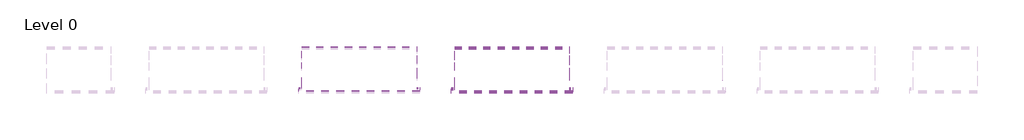
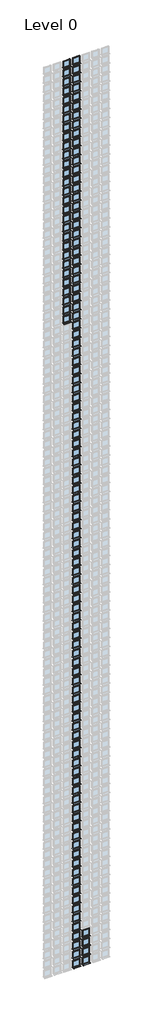
# One storey, part 12 of 75: 133 windows.
# Revit data of these elements (continued)
# Project information
#   Project Issue Date = "Issue Date"
#   Project Status = "Project Status"
#   Client Name = "Owner"
#   Project Address = "Enter address here"
#   Project Name = "Project Name"
#   Project Number = "Project Number"
# Type "Windows_Sgl_Plain : Square Green"
#   Type Mark = "51"
#   Operation = "SinglePanel"
#   Construction Type Id = "SGL"
#   Manufacturer = "Revit"
#   Keynote = "L10"
#   Analytic Construction = "Large single-glazed windows"
#   Wrap Layers (Ext) from Ext = 102.5 mm
#   Wrap Layers (Int) from Ext = 177.5 mm
#   Window Board Projection = 25 mm
#   Window Board Extension = 25 mm
#   Visual Light Transmittance = 0.9
#   Solar Heat Gain Coefficient = 0.86
#   Rough Width = 910 mm
#   Rough Height = 910 mm
#   Height = 910 mm
#   Width = 910 mm
#   Heat Transfer Coefficient (U) = 5.5617 W/(m²·K)
#   Glazing Thickness = 24 mm
#   FrameOffset - External = 50 mm
#   Frame Depth = 65 mm
#   Default Head Height = 2110 mm
#   Cill Depth = 87.5 mm
#   Cavity Closer Width = 50 mm
#   Cavity Closer Offset from Ext = 102.5 mm
#   Cavity Closer Depth = 85 mm
#   Vis - Cavity Closers = yes
#   Material Trim = Window Frame
#   Material Glass = Green Glass
#   Material Frame = Window Frame
#   Wall Closure = (empty or 0)
# Type "Windows_Sgl_Plain : Square Normal"
#   Type Mark = "44"
#   Operation = "SinglePanel"
#   Construction Type Id = "SGL"
#   Manufacturer = "Revit"
#   Keynote = "L10"
#   Analytic Construction = "Large single-glazed windows"
#   Wrap Layers (Ext) from Ext = 102.5 mm
#   Wrap Layers (Int) from Ext = 177.5 mm
#   Window Board Projection = 25 mm
#   Window Board Extension = 25 mm
#   Visual Light Transmittance = 0.9
#   Solar Heat Gain Coefficient = 0.86
#   Rough Width = 910 mm
#   Rough Height = 910 mm
#   Height = 910 mm
#   Width = 910 mm
#   Heat Transfer Coefficient (U) = 5.5617 W/(m²·K)
#   Glazing Thickness = 24 mm
#   FrameOffset - External = 50 mm
#   Frame Depth = 65 mm
#   Default Head Height = 2110 mm
#   Cill Depth = 87.5 mm
#   Cavity Closer Width = 50 mm
#   Cavity Closer Offset from Ext = 102.5 mm
#   Cavity Closer Depth = 85 mm
#   Vis - Cavity Closers = yes
#   Material Trim = Window Frame
#   Material Glass = Glass
#   Material Frame = Window Frame
#   Wall Closure = (empty or 0)
# Type "Windows_Sgl_Plain : Square Red"
#   Type Mark = "50"
#   Operation = "SinglePanel"
#   Construction Type Id = "SGL"
#   Manufacturer = "Revit"
#   Keynote = "L10"
#   Analytic Construction = "Large single-glazed windows"
#   Wrap Layers (Ext) from Ext = 102.5 mm
#   Wrap Layers (Int) from Ext = 177.5 mm
#   Window Board Projection = 25 mm
#   Window Board Extension = 25 mm
#   Visual Light Transmittance = 0.9
#   Solar Heat Gain Coefficient = 0.86
#   Rough Width = 910 mm
#   Rough Height = 910 mm
#   Height = 910 mm
#   Width = 910 mm
#   Heat Transfer Coefficient (U) = 5.5617 W/(m²·K)
#   Glazing Thickness = 24 mm
#   FrameOffset - External = 50 mm
#   Frame Depth = 65 mm
#   Default Head Height = 2110 mm
#   Cill Depth = 87.5 mm
#   Cavity Closer Width = 50 mm
#   Cavity Closer Offset from Ext = 102.5 mm
#   Cavity Closer Depth = 85 mm
#   Vis - Cavity Closers = yes
#   Material Trim = Window Frame
#   Material Glass = Red Glass
#   Material Frame = Window Frame
#   Wall Closure = (empty or 0)
# Element 1 (IfcWindow, "Windows_Sgl_Plain : Square Green")
#   Mark = "6458"
#   Phase Created = New Construction
#   Materials on its faces: "Window Frame", "Green Glass"
# Element 2 (IfcWindow, "Windows_Sgl_Plain : Square Green")
#   Mark = "12457"
#   Phase Created = New Construction
#   Materials on its faces: "Window Frame", "Green Glass"
# Element 3 (IfcWindow, "Windows_Sgl_Plain : Square Green")
#   Mark = "12557"
#   Phase Created = New Construction
#   Materials on its faces: "Window Frame", "Green Glass"
# Element 4 (IfcWindow, "Windows_Sgl_Plain : Square Normal")
#   Mark = "6457"
#   Phase Created = New Construction
#   Materials on its faces: "Window Frame", "Glass"
# Element 5 (IfcWindow, "Windows_Sgl_Plain : Square Normal")
#   Mark = "6557"
#   Phase Created = New Construction
#   Materials on its faces: "Window Frame", "Glass"
# Element 6 (IfcWindow, "Windows_Sgl_Plain : Square Normal")
#   Mark = "6558"
#   Phase Created = New Construction
#   Materials on its faces: "Window Frame", "Glass"
# Element 7 (IfcWindow, "Windows_Sgl_Plain : Square Normal")
#   Mark = "6657"
#   Phase Created = New Construction
#   Materials on its faces: "Window Frame", "Glass"
# Element 8 (IfcWindow, "Windows_Sgl_Plain : Square Normal")
#   Mark = "6757"
#   Phase Created = New Construction
#   Materials on its faces: "Window Frame", "Glass"
# Element 9 (IfcWindow, "Windows_Sgl_Plain : Square Normal")
#   Mark = "6857"
#   Phase Created = New Construction
#   Materials on its faces: "Window Frame", "Glass"
# Element 10 (IfcWindow, "Windows_Sgl_Plain : Square Normal")
#   Mark = "6957"
#   Phase Created = New Construction
#   Materials on its faces: "Window Frame", "Glass"
# Element 11 (IfcWindow, "Windows_Sgl_Plain : Square Normal")
#   Mark = "7057"
#   Phase Created = New Construction
#   Materials on its faces: "Window Frame", "Glass"
# Element 12 (IfcWindow, "Windows_Sgl_Plain : Square Normal")
#   Mark = "7157"
#   Phase Created = New Construction
#   Materials on its faces: "Window Frame", "Glass"
# Element 13 (IfcWindow, "Windows_Sgl_Plain : Square Normal")
#   Mark = "7257"
#   Phase Created = New Construction
#   Materials on its faces: "Window Frame", "Glass"
# Element 14 (IfcWindow, "Windows_Sgl_Plain : Square Normal")
#   Mark = "7357"
#   Phase Created = New Construction
#   Materials on its faces: "Window Frame", "Glass"
# Element 15 (IfcWindow, "Windows_Sgl_Plain : Square Normal")
#   Mark = "7457"
#   Phase Created = New Construction
#   Materials on its faces: "Window Frame", "Glass"
# Element 16 (IfcWindow, "Windows_Sgl_Plain : Square Normal")
#   Mark = "7557"
#   Phase Created = New Construction
#   Materials on its faces: "Window Frame", "Glass"
# Element 17 (IfcWindow, "Windows_Sgl_Plain : Square Normal")
#   Mark = "7657"
#   Phase Created = New Construction
#   Materials on its faces: "Window Frame", "Glass"
# Element 18 (IfcWindow, "Windows_Sgl_Plain : Square Normal")
#   Mark = "7757"
#   Phase Created = New Construction
#   Materials on its faces: "Window Frame", "Glass"
# Element 19 (IfcWindow, "Windows_Sgl_Plain : Square Normal")
#   Mark = "7857"
#   Phase Created = New Construction
#   Materials on its faces: "Window Frame", "Glass"
# Element 20 (IfcWindow, "Windows_Sgl_Plain : Square Normal")
#   Mark = "7957"
#   Phase Created = New Construction
#   Materials on its faces: "Window Frame", "Glass"
# Element 21 (IfcWindow, "Windows_Sgl_Plain : Square Normal")
#   Mark = "8057"
#   Phase Created = New Construction
#   Materials on its faces: "Window Frame", "Glass"
# Element 22 (IfcWindow, "Windows_Sgl_Plain : Square Normal")
#   Mark = "8157"
#   Phase Created = New Construction
#   Materials on its faces: "Window Frame", "Glass"
# Element 23 (IfcWindow, "Windows_Sgl_Plain : Square Normal")
#   Mark = "8257"
#   Phase Created = New Construction
#   Materials on its faces: "Window Frame", "Glass"
# Element 24 (IfcWindow, "Windows_Sgl_Plain : Square Normal")
#   Mark = "8357"
#   Phase Created = New Construction
#   Materials on its faces: "Window Frame", "Glass"
# Element 25 (IfcWindow, "Windows_Sgl_Plain : Square Normal")
#   Mark = "8457"
#   Phase Created = New Construction
#   Materials on its faces: "Window Frame", "Glass"
# Element 26 (IfcWindow, "Windows_Sgl_Plain : Square Normal")
#   Mark = "8557"
#   Phase Created = New Construction
#   Materials on its faces: "Window Frame", "Glass"
# Element 27 (IfcWindow, "Windows_Sgl_Plain : Square Normal")
#   Mark = "8657"
#   Phase Created = New Construction
#   Materials on its faces: "Window Frame", "Glass"
# Element 28 (IfcWindow, "Windows_Sgl_Plain : Square Normal")
#   Mark = "8757"
#   Phase Created = New Construction
#   Materials on its faces: "Window Frame", "Glass"
# Element 29 (IfcWindow, "Windows_Sgl_Plain : Square Normal")
#   Mark = "8857"
#   Phase Created = New Construction
#   Materials on its faces: "Window Frame", "Glass"
# Element 30 (IfcWindow, "Windows_Sgl_Plain : Square Normal")
#   Mark = "8957"
#   Phase Created = New Construction
#   Materials on its faces: "Window Frame", "Glass"
# Element 31 (IfcWindow, "Windows_Sgl_Plain : Square Normal")
#   Mark = "9057"
#   Phase Created = New Construction
#   Materials on its faces: "Window Frame", "Glass"
# Element 32 (IfcWindow, "Windows_Sgl_Plain : Square Normal")
#   Mark = "9157"
#   Phase Created = New Construction
#   Materials on its faces: "Window Frame", "Glass"
# Element 33 (IfcWindow, "Windows_Sgl_Plain : Square Normal")
#   Mark = "9257"
#   Phase Created = New Construction
#   Materials on its faces: "Window Frame", "Glass"
# Element 34 (IfcWindow, "Windows_Sgl_Plain : Square Normal")
#   Mark = "9357"
#   Phase Created = New Construction
#   Materials on its faces: "Window Frame", "Glass"
# Element 35 (IfcWindow, "Windows_Sgl_Plain : Square Normal")
#   Mark = "9457"
#   Phase Created = New Construction
#   Materials on its faces: "Window Frame", "Glass"
# Element 36 (IfcWindow, "Windows_Sgl_Plain : Square Normal")
#   Mark = "9557"
#   Phase Created = New Construction
#   Materials on its faces: "Window Frame", "Glass"
# Element 37 (IfcWindow, "Windows_Sgl_Plain : Square Normal")
#   Mark = "9657"
#   Phase Created = New Construction
#   Materials on its faces: "Window Frame", "Glass"
# Element 38 (IfcWindow, "Windows_Sgl_Plain : Square Normal")
#   Mark = "9757"
#   Phase Created = New Construction
#   Materials on its faces: "Window Frame", "Glass"
# Element 39 (IfcWindow, "Windows_Sgl_Plain : Square Normal")
#   Mark = "9857"
#   Phase Created = New Construction
#   Materials on its faces: "Window Frame", "Glass"
# Element 40 (IfcWindow, "Windows_Sgl_Plain : Square Normal")
#   Mark = "9957"
#   Phase Created = New Construction
#   Materials on its faces: "Window Frame", "Glass"
# Element 41 (IfcWindow, "Windows_Sgl_Plain : Square Normal")
#   Mark = "10057"
#   Phase Created = New Construction
#   Materials on its faces: "Window Frame", "Glass"
# Element 42 (IfcWindow, "Windows_Sgl_Plain : Square Normal")
#   Mark = "10157"
#   Phase Created = New Construction
#   Materials on its faces: "Window Frame", "Glass"
# Element 43 (IfcWindow, "Windows_Sgl_Plain : Square Normal")
#   Mark = "10257"
#   Phase Created = New Construction
#   Materials on its faces: "Window Frame", "Glass"
# Element 44 (IfcWindow, "Windows_Sgl_Plain : Square Normal")
#   Mark = "10357"
#   Phase Created = New Construction
#   Materials on its faces: "Window Frame", "Glass"
# Element 45 (IfcWindow, "Windows_Sgl_Plain : Square Normal")
#   Mark = "10457"
#   Phase Created = New Construction
#   Materials on its faces: "Window Frame", "Glass"
# Element 46 (IfcWindow, "Windows_Sgl_Plain : Square Normal")
#   Mark = "10557"
#   Phase Created = New Construction
#   Materials on its faces: "Window Frame", "Glass"
# Element 47 (IfcWindow, "Windows_Sgl_Plain : Square Normal")
#   Mark = "11057"
#   Phase Created = New Construction
#   Materials on its faces: "Window Frame", "Glass"
# Element 48 (IfcWindow, "Windows_Sgl_Plain : Square Normal")
#   Mark = "11157"
#   Phase Created = New Construction
#   Materials on its faces: "Window Frame", "Glass"
# Element 49 (IfcWindow, "Windows_Sgl_Plain : Square Normal")
#   Mark = "11257"
#   Phase Created = New Construction
#   Materials on its faces: "Window Frame", "Glass"
# Element 50 (IfcWindow, "Windows_Sgl_Plain : Square Normal")
#   Mark = "11357"
#   Phase Created = New Construction
#   Materials on its faces: "Window Frame", "Glass"
# Element 51 (IfcWindow, "Windows_Sgl_Plain : Square Normal")
#   Mark = "11457"
#   Phase Created = New Construction
#   Materials on its faces: "Window Frame", "Glass"
# Element 52 (IfcWindow, "Windows_Sgl_Plain : Square Normal")
#   Mark = "11557"
#   Phase Created = New Construction
#   Materials on its faces: "Window Frame", "Glass"
# Element 53 (IfcWindow, "Windows_Sgl_Plain : Square Normal")
#   Mark = "11657"
#   Phase Created = New Construction
#   Materials on its faces: "Window Frame", "Glass"
# Element 54 (IfcWindow, "Windows_Sgl_Plain : Square Normal")
#   Mark = "11757"
#   Phase Created = New Construction
#   Materials on its faces: "Window Frame", "Glass"
# Element 55 (IfcWindow, "Windows_Sgl_Plain : Square Normal")
#   Mark = "11857"
#   Phase Created = New Construction
#   Materials on its faces: "Window Frame", "Glass"
# Element 56 (IfcWindow, "Windows_Sgl_Plain : Square Normal")
#   Mark = "11957"
#   Phase Created = New Construction
#   Materials on its faces: "Window Frame", "Glass"
# Element 57 (IfcWindow, "Windows_Sgl_Plain : Square Normal")
#   Mark = "12057"
#   Phase Created = New Construction
#   Materials on its faces: "Window Frame", "Glass"
# Element 58 (IfcWindow, "Windows_Sgl_Plain : Square Normal")
#   Mark = "12157"
#   Phase Created = New Construction
#   Materials on its faces: "Window Frame", "Glass"
# Element 59 (IfcWindow, "Windows_Sgl_Plain : Square Normal")
#   Mark = "12257"
#   Phase Created = New Construction
#   Materials on its faces: "Window Frame", "Glass"
# Element 60 (IfcWindow, "Windows_Sgl_Plain : Square Normal")
#   Mark = "12357"
#   Phase Created = New Construction
#   Materials on its faces: "Window Frame", "Glass"
# Element 61 (IfcWindow, "Windows_Sgl_Plain : Square Normal")
#   Mark = "12657"
#   Phase Created = New Construction
#   Materials on its faces: "Window Frame", "Glass"
# Element 62 (IfcWindow, "Windows_Sgl_Plain : Square Normal")
#   Mark = "12757"
#   Phase Created = New Construction
#   Materials on its faces: "Window Frame", "Glass"
# Element 63 (IfcWindow, "Windows_Sgl_Plain : Square Normal")
#   Mark = "12857"
#   Phase Created = New Construction
#   Materials on its faces: "Window Frame", "Glass"
# Element 64 (IfcWindow, "Windows_Sgl_Plain : Square Normal")
#   Mark = "12957"
#   Phase Created = New Construction
#   Materials on its faces: "Window Frame", "Glass"
# Element 65 (IfcWindow, "Windows_Sgl_Plain : Square Normal")
#   Mark = "13057"
#   Phase Created = New Construction
#   Materials on its faces: "Window Frame", "Glass"
# Element 66 (IfcWindow, "Windows_Sgl_Plain : Square Normal")
#   Mark = "13157"
#   Phase Created = New Construction
#   Materials on its faces: "Window Frame", "Glass"
# Element 67 (IfcWindow, "Windows_Sgl_Plain : Square Normal")
#   Mark = "13257"
#   Phase Created = New Construction
#   Materials on its faces: "Window Frame", "Glass"
# Element 68 (IfcWindow, "Windows_Sgl_Plain : Square Normal")
#   Mark = "13356"
#   Phase Created = New Construction
#   Materials on its faces: "Window Frame", "Glass"
# Element 69 (IfcWindow, "Windows_Sgl_Plain : Square Normal")
#   Mark = "13357"
#   Phase Created = New Construction
#   Materials on its faces: "Window Frame", "Glass"
# Element 70 (IfcWindow, "Windows_Sgl_Plain : Square Normal")
#   Mark = "13456"
#   Phase Created = New Construction
#   Materials on its faces: "Window Frame", "Glass"
# Element 71 (IfcWindow, "Windows_Sgl_Plain : Square Normal")
#   Mark = "13457"
#   Phase Created = New Construction
#   Materials on its faces: "Window Frame", "Glass"
# Element 72 (IfcWindow, "Windows_Sgl_Plain : Square Normal")
#   Mark = "13556"
#   Phase Created = New Construction
#   Materials on its faces: "Window Frame", "Glass"
# Element 73 (IfcWindow, "Windows_Sgl_Plain : Square Normal")
#   Mark = "13557"
#   Phase Created = New Construction
#   Materials on its faces: "Window Frame", "Glass"
# Element 74 (IfcWindow, "Windows_Sgl_Plain : Square Normal")
#   Mark = "13656"
#   Phase Created = New Construction
#   Materials on its faces: "Window Frame", "Glass"
# Element 75 (IfcWindow, "Windows_Sgl_Plain : Square Normal")
#   Mark = "13657"
#   Phase Created = New Construction
#   Materials on its faces: "Window Frame", "Glass"
# Element 76 (IfcWindow, "Windows_Sgl_Plain : Square Normal")
#   Mark = "13756"
#   Phase Created = New Construction
#   Materials on its faces: "Window Frame", "Glass"
# Element 77 (IfcWindow, "Windows_Sgl_Plain : Square Normal")
#   Mark = "13757"
#   Phase Created = New Construction
#   Materials on its faces: "Window Frame", "Glass"
# Element 78 (IfcWindow, "Windows_Sgl_Plain : Square Normal")
#   Mark = "13856"
#   Phase Created = New Construction
#   Materials on its faces: "Window Frame", "Glass"
# Element 79 (IfcWindow, "Windows_Sgl_Plain : Square Normal")
#   Mark = "13857"
#   Phase Created = New Construction
#   Materials on its faces: "Window Frame", "Glass"
# Element 80 (IfcWindow, "Windows_Sgl_Plain : Square Normal")
#   Mark = "13956"
#   Phase Created = New Construction
#   Materials on its faces: "Window Frame", "Glass"
# Element 81 (IfcWindow, "Windows_Sgl_Plain : Square Normal")
#   Mark = "13957"
#   Phase Created = New Construction
#   Materials on its faces: "Window Frame", "Glass"
# Element 82 (IfcWindow, "Windows_Sgl_Plain : Square Normal")
#   Mark = "14056"
#   Phase Created = New Construction
#   Materials on its faces: "Window Frame", "Glass"
# Element 83 (IfcWindow, "Windows_Sgl_Plain : Square Normal")
#   Mark = "14057"
#   Phase Created = New Construction
#   Materials on its faces: "Window Frame", "Glass"
# Element 84 (IfcWindow, "Windows_Sgl_Plain : Square Normal")
#   Mark = "14156"
#   Phase Created = New Construction
#   Materials on its faces: "Window Frame", "Glass"
# Element 85 (IfcWindow, "Windows_Sgl_Plain : Square Normal")
#   Mark = "14157"
#   Phase Created = New Construction
#   Materials on its faces: "Window Frame", "Glass"
# Element 86 (IfcWindow, "Windows_Sgl_Plain : Square Normal")
#   Mark = "14256"
#   Phase Created = New Construction
#   Materials on its faces: "Window Frame", "Glass"
# Element 87 (IfcWindow, "Windows_Sgl_Plain : Square Normal")
#   Mark = "14257"
#   Phase Created = New Construction
#   Materials on its faces: "Window Frame", "Glass"
# Element 88 (IfcWindow, "Windows_Sgl_Plain : Square Normal")
#   Mark = "14356"
#   Phase Created = New Construction
#   Materials on its faces: "Window Frame", "Glass"
# Element 89 (IfcWindow, "Windows_Sgl_Plain : Square Normal")
#   Mark = "14357"
#   Phase Created = New Construction
#   Materials on its faces: "Window Frame", "Glass"
# Element 90 (IfcWindow, "Windows_Sgl_Plain : Square Normal")
#   Mark = "14456"
#   Phase Created = New Construction
#   Materials on its faces: "Window Frame", "Glass"
# Element 91 (IfcWindow, "Windows_Sgl_Plain : Square Normal")
#   Mark = "14457"
#   Phase Created = New Construction
#   Materials on its faces: "Window Frame", "Glass"
# Element 92 (IfcWindow, "Windows_Sgl_Plain : Square Normal")
#   Mark = "14556"
#   Phase Created = New Construction
#   Materials on its faces: "Window Frame", "Glass"
# Element 93 (IfcWindow, "Windows_Sgl_Plain : Square Normal")
#   Mark = "14557"
#   Phase Created = New Construction
#   Materials on its faces: "Window Frame", "Glass"
# Element 94 (IfcWindow, "Windows_Sgl_Plain : Square Normal")
#   Mark = "14656"
#   Phase Created = New Construction
#   Materials on its faces: "Window Frame", "Glass"
# Element 95 (IfcWindow, "Windows_Sgl_Plain : Square Normal")
#   Mark = "14657"
#   Phase Created = New Construction
#   Materials on its faces: "Window Frame", "Glass"
# Element 96 (IfcWindow, "Windows_Sgl_Plain : Square Normal")
#   Mark = "14756"
#   Phase Created = New Construction
#   Materials on its faces: "Window Frame", "Glass"
# Element 97 (IfcWindow, "Windows_Sgl_Plain : Square Normal")
#   Mark = "14757"
#   Phase Created = New Construction
#   Materials on its faces: "Window Frame", "Glass"
# Element 98 (IfcWindow, "Windows_Sgl_Plain : Square Normal")
#   Mark = "14856"
#   Phase Created = New Construction
#   Materials on its faces: "Window Frame", "Glass"
# Element 99 (IfcWindow, "Windows_Sgl_Plain : Square Normal")
#   Mark = "14857"
#   Phase Created = New Construction
#   Materials on its faces: "Window Frame", "Glass"
# Element 100 (IfcWindow, "Windows_Sgl_Plain : Square Normal")
#   Mark = "14956"
#   Phase Created = New Construction
#   Materials on its faces: "Window Frame", "Glass"
# Element 101 (IfcWindow, "Windows_Sgl_Plain : Square Normal")
#   Mark = "14957"
#   Phase Created = New Construction
#   Materials on its faces: "Window Frame", "Glass"
# Element 102 (IfcWindow, "Windows_Sgl_Plain : Square Normal")
#   Mark = "15056"
#   Phase Created = New Construction
#   Materials on its faces: "Window Frame", "Glass"
# Element 103 (IfcWindow, "Windows_Sgl_Plain : Square Normal")
#   Mark = "15057"
#   Phase Created = New Construction
#   Materials on its faces: "Window Frame", "Glass"
# Element 104 (IfcWindow, "Windows_Sgl_Plain : Square Normal")
#   Mark = "15156"
#   Phase Created = New Construction
#   Materials on its faces: "Window Frame", "Glass"
# Element 105 (IfcWindow, "Windows_Sgl_Plain : Square Normal")
#   Mark = "15157"
#   Phase Created = New Construction
#   Materials on its faces: "Window Frame", "Glass"
# Element 106 (IfcWindow, "Windows_Sgl_Plain : Square Normal")
#   Mark = "15256"
#   Phase Created = New Construction
#   Materials on its faces: "Window Frame", "Glass"
# Element 107 (IfcWindow, "Windows_Sgl_Plain : Square Normal")
#   Mark = "15257"
#   Phase Created = New Construction
#   Materials on its faces: "Window Frame", "Glass"
# Element 108 (IfcWindow, "Windows_Sgl_Plain : Square Normal")
#   Mark = "15356"
#   Phase Created = New Construction
#   Materials on its faces: "Window Frame", "Glass"
# Element 109 (IfcWindow, "Windows_Sgl_Plain : Square Normal")
#   Mark = "15357"
#   Phase Created = New Construction
#   Materials on its faces: "Window Frame", "Glass"
# Element 110 (IfcWindow, "Windows_Sgl_Plain : Square Normal")
#   Mark = "15456"
#   Phase Created = New Construction
#   Materials on its faces: "Window Frame", "Glass"
# Element 111 (IfcWindow, "Windows_Sgl_Plain : Square Normal")
#   Mark = "15457"
#   Phase Created = New Construction
#   Materials on its faces: "Window Frame", "Glass"
# Element 112 (IfcWindow, "Windows_Sgl_Plain : Square Normal")
#   Mark = "15556"
#   Phase Created = New Construction
#   Materials on its faces: "Window Frame", "Glass"
# Element 113 (IfcWindow, "Windows_Sgl_Plain : Square Normal")
#   Mark = "15557"
#   Phase Created = New Construction
#   Materials on its faces: "Window Frame", "Glass"
# Element 114 (IfcWindow, "Windows_Sgl_Plain : Square Normal")
#   Mark = "15656"
#   Phase Created = New Construction
#   Materials on its faces: "Window Frame", "Glass"
# Element 115 (IfcWindow, "Windows_Sgl_Plain : Square Normal")
#   Mark = "15657"
#   Phase Created = New Construction
#   Materials on its faces: "Window Frame", "Glass"
# Element 116 (IfcWindow, "Windows_Sgl_Plain : Square Normal")
#   Mark = "15756"
#   Phase Created = New Construction
#   Materials on its faces: "Window Frame", "Glass"
# Element 117 (IfcWindow, "Windows_Sgl_Plain : Square Normal")
#   Mark = "15757"
#   Phase Created = New Construction
#   Materials on its faces: "Window Frame", "Glass"
# Element 118 (IfcWindow, "Windows_Sgl_Plain : Square Normal")
#   Mark = "15856"
#   Phase Created = New Construction
#   Materials on its faces: "Window Frame", "Glass"
# Element 119 (IfcWindow, "Windows_Sgl_Plain : Square Normal")
#   Mark = "15857"
#   Phase Created = New Construction
#   Materials on its faces: "Window Frame", "Glass"
# Element 120 (IfcWindow, "Windows_Sgl_Plain : Square Normal")
#   Mark = "15956"
#   Phase Created = New Construction
#   Materials on its faces: "Window Frame", "Glass"
# Element 121 (IfcWindow, "Windows_Sgl_Plain : Square Normal")
#   Mark = "15957"
#   Phase Created = New Construction
#   Materials on its faces: "Window Frame", "Glass"
# Element 122 (IfcWindow, "Windows_Sgl_Plain : Square Normal")
#   Mark = "16056"
#   Phase Created = New Construction
#   Materials on its faces: "Window Frame", "Glass"
# Element 123 (IfcWindow, "Windows_Sgl_Plain : Square Normal")
#   Mark = "16057"
#   Phase Created = New Construction
#   Materials on its faces: "Window Frame", "Glass"
# Element 124 (IfcWindow, "Windows_Sgl_Plain : Square Normal")
#   Mark = "16156"
#   Phase Created = New Construction
#   Materials on its faces: "Window Frame", "Glass"
# Element 125 (IfcWindow, "Windows_Sgl_Plain : Square Normal")
#   Mark = "16157"
#   Phase Created = New Construction
#   Materials on its faces: "Window Frame", "Glass"
# Element 126 (IfcWindow, "Windows_Sgl_Plain : Square Red")
#   Mark = "6257"
#   Phase Created = New Construction
#   Materials on its faces: "Window Frame", "Red Glass"
# Element 127 (IfcWindow, "Windows_Sgl_Plain : Square Red")
#   Mark = "6258"
#   Phase Created = New Construction
#   Materials on its faces: "Window Frame", "Red Glass"
# Element 128 (IfcWindow, "Windows_Sgl_Plain : Square Red")
#   Mark = "6357"
#   Phase Created = New Construction
#   Materials on its faces: "Window Frame", "Red Glass"
# Element 129 (IfcWindow, "Windows_Sgl_Plain : Square Red")
#   Mark = "6358"
#   Phase Created = New Construction
#   Materials on its faces: "Window Frame", "Red Glass"
# Element 130 (IfcWindow, "Windows_Sgl_Plain : Square Red")
#   Mark = "10657"
#   Phase Created = New Construction
#   Materials on its faces: "Window Frame", "Red Glass"
# Element 131 (IfcWindow, "Windows_Sgl_Plain : Square Red")
#   Mark = "10757"
#   Phase Created = New Construction
#   Materials on its faces: "Window Frame", "Red Glass"
# Element 132 (IfcWindow, "Windows_Sgl_Plain : Square Red")
#   Mark = "10857"
#   Phase Created = New Construction
#   Materials on its faces: "Window Frame", "Red Glass"
# Element 133 (IfcWindow, "Windows_Sgl_Plain : Square Red")
#   Mark = "10957"
#   Phase Created = New Construction
#   Materials on its faces: "Window Frame", "Red Glass"
# Materials
#   "Window Frame": class "Miscellaneous", colour RGB 249 249 249, transparency 0, Keynote = "L10", Cost = 0
#   "Green Glass": class "Glass", colour RGB 0 242 0, transparency 0.8, Description = "Soda Lime Glass", Cost = 0
#   "Glass": class "Glass", colour RGB 62 67 255, transparency 0.85, Description = "Soda Lime Glass", Cost = 0
#   "Red Glass": class "Glass", colour RGB 255 83 83, transparency 0.85, Description = "Soda Lime Glass", Cost = 0
